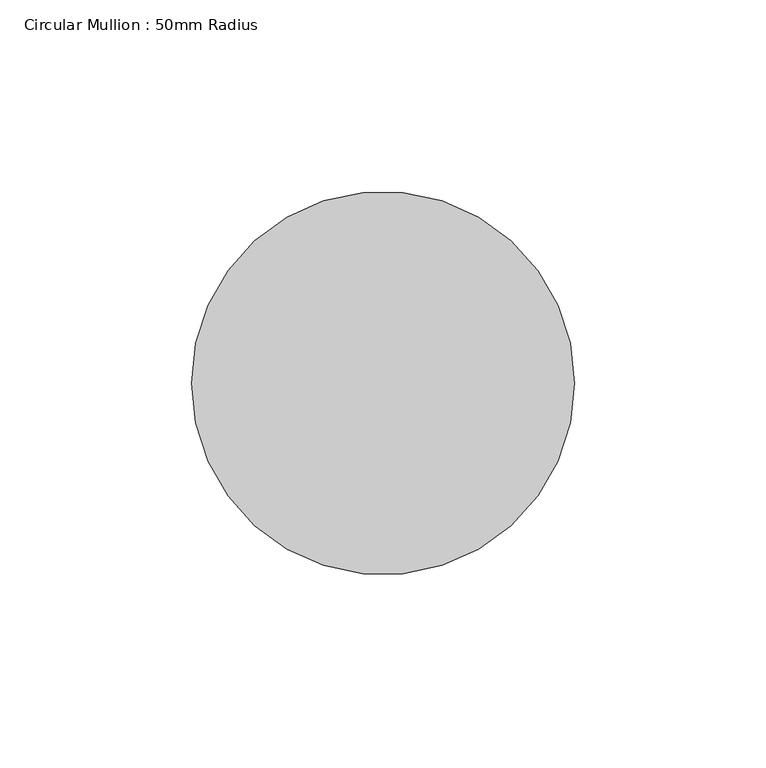
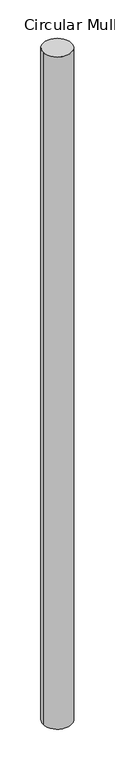
"""IFC4 building model written with IfcOpenShell, lengths in millimetres: member geometry, Circular Mullion : 50mm Radius."""

from ifc_helpers import new_model, si_unit, point, frame, origin, origin_2d, place, context, project, spatial, circle_curve, trimmed, segment, composite_curve, outline, extrude, source, transform, mapped, element, save


def circular_mullion_50mm_radius_f7d91639(model_context):
    return source(origin(), model_context, "Body", "SweptSolid", [
        extrude(outline(composite_curve([segment(trimmed(circle_curve(origin_2d(), 50.0), [point((50.0, 0.0))], [point((-50.0, 0.0))], False, "CARTESIAN"), True, "CONTINUOUS"), segment(trimmed(circle_curve(origin_2d(), 50.0), [point((-50.0, 0.0))], [point((50.0, 0.0))], False, "CARTESIAN"), True, "CONTINUOUS")], self_intersect=False)), frame((0.0, 0.0, -2507.5632055), z_axis=(0.0, 0.0, 1.0), x_axis=(1.0, 0.0, 0.0)), (0.0, 0.0, 1.0), 2507.5632055),
    ])


if __name__ == "__main__":
    model = new_model("IFC4")
    model_context = context("Model", 3, world=origin())
    ifc_project = project(units=[si_unit("LENGTHUNIT", "METRE", prefix="MILLI")], contexts=[model_context])
    site = spatial("IfcSite", under=ifc_project)
    building = spatial("IfcBuilding", under=site)
    placement = place(None, origin())
    circular_mullion_50mm_radius_shape = circular_mullion_50mm_radius_f7d91639(model_context)
    element("IfcMember", 1, ObjectType="Circular Mullion : 50mm Radius", at=placement, inside=building, context=model_context, shape_type="MappedRepresentation", body=[
        mapped(circular_mullion_50mm_radius_shape, transform((0.0, 0.0, 0.0), x_axis=(1.0, 0.0, 0.0), y_axis=(0.0, 1.0, 0.0), z_axis=(0.0, 0.0, 1.0))),
    ])
    save(model, "model.ifc")

# Revit data of these elements
# Type "Circular Mullion : 50mm Radius"
#   built-in parameter 1007350 = 0.164042 (stored number, unit not read)
# Element 1 (IfcMember, "Circular Mullion : 50mm Radius")
#   Materials on its faces: "Aluminium"
# Materials
#   "Aluminium": class "Metal", colour RGB 247 247 247, transparency 0, Description = "Aluminium 6061", Cost = 0
